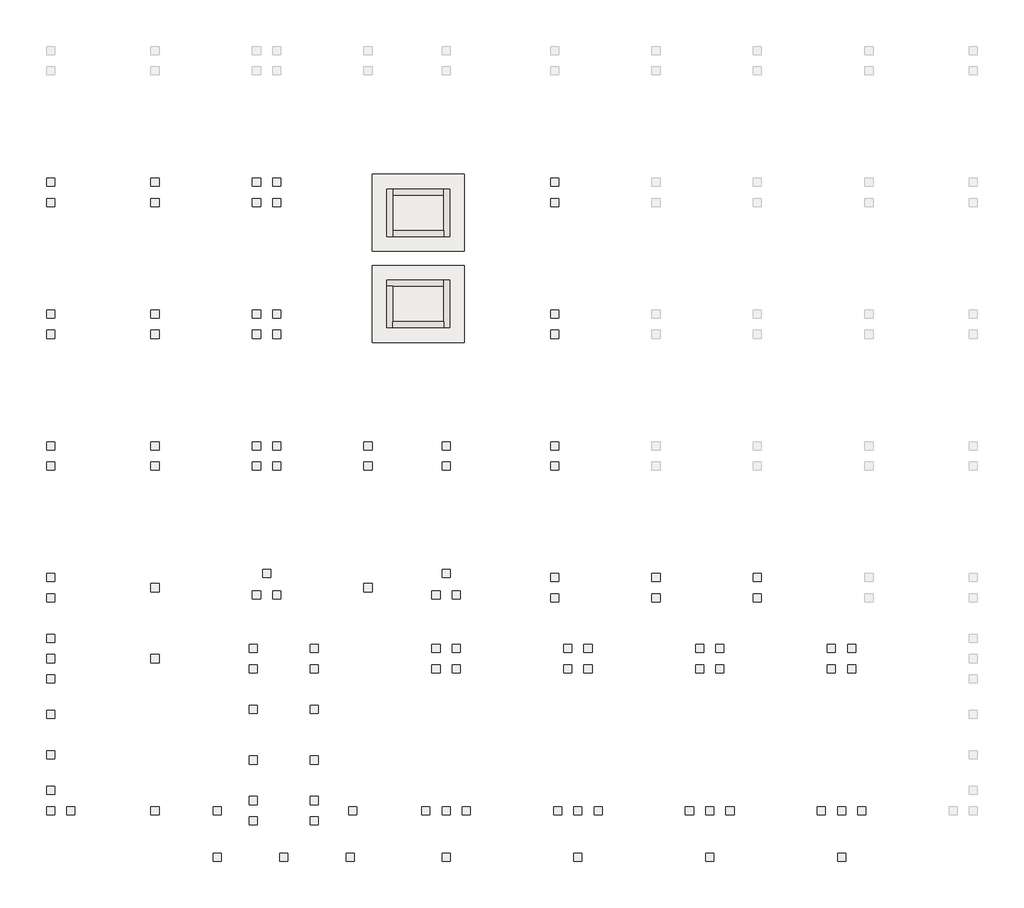
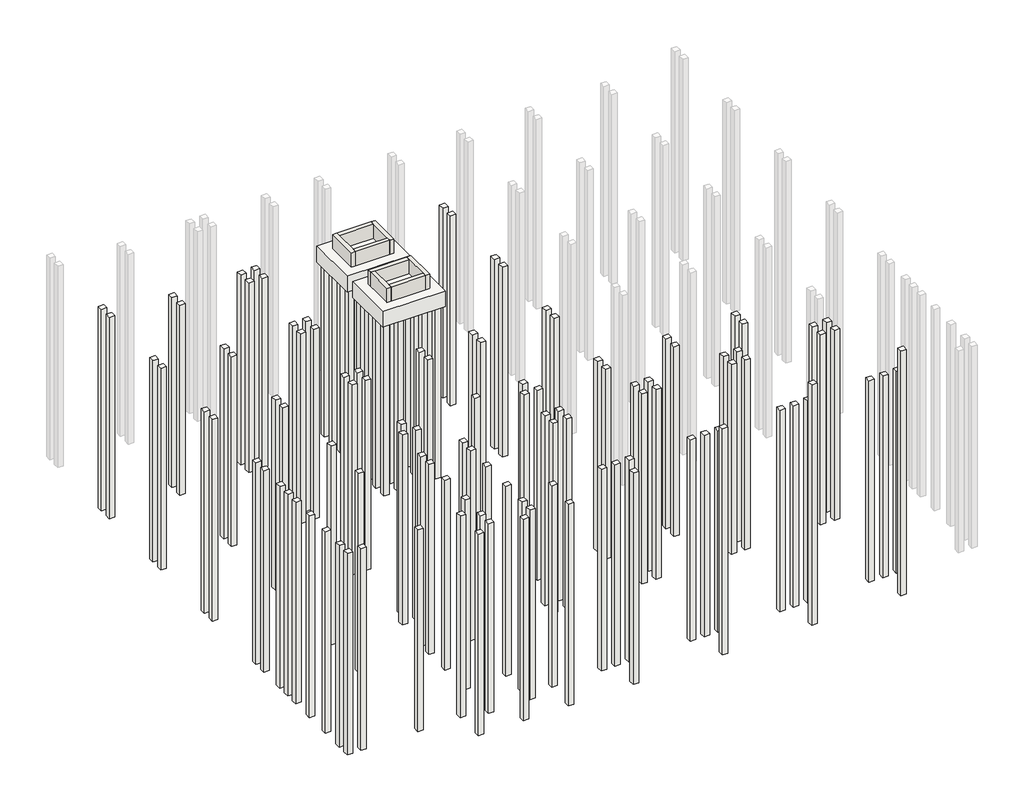
# Not in any storey, part 1 of 2: 143 slabs, 8 walls.
# Revit data of these elements (continued)
# Type "NLRS_16_SFO_LB_funderingspoer meerpaals beton ihwg-MMBC-SH_gen_rsf : funderingspoer beton ihwg_gen__lift bxlxh 3800x4550x1200" (continued)
#   Structural Material = NLRS_f2_beton ihwg_gen_rsf
#   Keynote = ""
# Type "NLRS_17_SFO_TLB_funderingspaal geheid beton prefab-AV-MMBPC_gen_rsf : heipaal beton prefab_gen__bxh 400x400"
#   Export Type to IFC As = "IfcPile"
#   Type IfcGUID = "10$Kfo5uPCAOPJEOo5LE_W"
#   Type Comments = "prefab heipaal 400x400"
#   Model = " "
#   Manufacturer = " "
#   Description = "prefab heipaal 400x400"
#   Assembly Code = "17.21"
#   Width = 400 mm
#   Slanted Angle [instance default] = 0.00°
#   NLRS_S_draagvermogen_trek [instance default] = 0.00 kN
#   NLRS_S_draagvermogen_druk [instance default] = 0.00 kN
#   NLRS_C_lengte [instance default] = 1660 mm
#   NLRS_C_hoogte = 400 mm
#   NLRS_C_breedte = 400 mm
#   Height [instance default] = 1660 mm
#   Length [instance default] = 1660 mm
#   Angle [instance default] = 0.00°
#   Slanted [instance default] = 0
#   Structural Material = NLRS_f2_beton prefab_gen_rsf
#   Keynote = ""
# Type "NLRS_16_WA_beton ihw 300_gen_rsf"
#   Keynote = ""
#   Export Type to IFC As = "IfcWall"
#   Type IfcGUID = "3S1HfGygHC08_ZXeiJ7DHR"
#   Description = "buitenwand beton ihw, generiek"
#   Assembly Code = "16.23"
#   Layers, outside or top first: 300 mm "NLRS_f2_beton ihwg_gen_rsf" (function 1)
# Element 1 (IfcSlab, "NLRS_16_SFO_LB_funderingspoer meerpaals beton ihwg-MMBC-SH_gen_rsf : funderingspoer beton ihwg_gen__lift bxlxh 3800x4550x1200")
#   IfcGUID = "22y6L5gAz9AR8RjJaZzOwK"
#   Height = 1200 mm
#   Depth = 0 mm
#   IsExternal = yes
#   LoadBearing = yes
#   Phase Created = NLRS_nieuw
#   Materials on its faces: "NLRS_f2_beton ihwg_gen_rsf"
# Element 2 (IfcSlab, "NLRS_16_SFO_LB_funderingspoer meerpaals beton ihwg-MMBC-SH_gen_rsf : funderingspoer beton ihwg_gen__lift bxlxh 3800x4550x1200")
#   IfcGUID = "22y6L5gAz9AR8RjJaZzOui"
#   Height = 1200 mm
#   Depth = 0 mm
#   IsExternal = yes
#   LoadBearing = yes
#   Phase Created = NLRS_nieuw
#   Materials on its faces: "NLRS_f2_beton ihwg_gen_rsf"
# Element 3 (IfcSlab, "NLRS_17_SFO_TLB_funderingspaal geheid beton prefab-AV-MMBPC_gen_rsf : heipaal beton prefab_gen__bxh 400x400")
#   IfcGUID = "10$Kfo5uPCAOPJEOo5LEvz"
#   Slanted Angle = 0.00°
#   NLRS_S_draagvermogen_trek = 0.00 kN
#   NLRS_S_draagvermogen_druk = 0.00 kN
#   Angle = 0.00°
#   IsExternal = yes
#   LoadBearing = yes
#   Slanted = 0
#   Phase Created = NLRS_nieuw
#   Materials on its faces: "NLRS_f2_beton prefab_gen_rsf"
# Element 4 (IfcSlab, "NLRS_17_SFO_TLB_funderingspaal geheid beton prefab-AV-MMBPC_gen_rsf : heipaal beton prefab_gen__bxh 400x400")
#   IfcGUID = "10$Kfo5uPCAOPJEOo5LEuK"
#   Slanted Angle = 0.00°
#   NLRS_S_draagvermogen_trek = 0.00 kN
#   NLRS_S_draagvermogen_druk = 0.00 kN
#   Angle = 0.00°
#   IsExternal = yes
#   LoadBearing = yes
#   Slanted = 0
#   Phase Created = NLRS_nieuw
#   Materials on its faces: "NLRS_f2_beton prefab_gen_rsf"
# Element 5 (IfcSlab, "NLRS_17_SFO_TLB_funderingspaal geheid beton prefab-AV-MMBPC_gen_rsf : heipaal beton prefab_gen__bxh 400x400")
#   IfcGUID = "10$Kfo5uPCAOPJEOo5LEuY"
#   Slanted Angle = 0.00°
#   NLRS_S_draagvermogen_trek = 0.00 kN
#   NLRS_S_draagvermogen_druk = 0.00 kN
#   Angle = 0.00°
#   IsExternal = yes
#   LoadBearing = yes
#   Slanted = 0
#   Phase Created = NLRS_nieuw
#   Materials on its faces: "NLRS_f2_beton prefab_gen_rsf"
# Element 6 (IfcSlab, "NLRS_17_SFO_TLB_funderingspaal geheid beton prefab-AV-MMBPC_gen_rsf : heipaal beton prefab_gen__bxh 400x400")
#   IfcGUID = "10$Kfo5uPCAOPJEOo5LEu$"
#   Slanted Angle = 0.00°
#   NLRS_S_draagvermogen_trek = 0.00 kN
#   NLRS_S_draagvermogen_druk = 0.00 kN
#   Angle = 0.00°
#   IsExternal = yes
#   LoadBearing = yes
#   Slanted = 0
#   Phase Created = NLRS_nieuw
#   Materials on its faces: "NLRS_f2_beton prefab_gen_rsf"
# Element 7 (IfcSlab, "NLRS_17_SFO_TLB_funderingspaal geheid beton prefab-AV-MMBPC_gen_rsf : heipaal beton prefab_gen__bxh 400x400")
#   IfcGUID = "10$Kfo5uPCAOPJEOo5LEun"
#   Slanted Angle = 0.00°
#   NLRS_S_draagvermogen_trek = 0.00 kN
#   NLRS_S_draagvermogen_druk = 0.00 kN
#   Angle = 0.00°
#   IsExternal = yes
#   LoadBearing = yes
#   Slanted = 0
#   Phase Created = NLRS_nieuw
#   Materials on its faces: "NLRS_f2_beton prefab_gen_rsf"
# Element 8 (IfcSlab, "NLRS_17_SFO_TLB_funderingspaal geheid beton prefab-AV-MMBPC_gen_rsf : heipaal beton prefab_gen__bxh 400x400")
#   IfcGUID = "10$Kfo5uPCAOPJEOo5LEtC"
#   Slanted Angle = 0.00°
#   NLRS_S_draagvermogen_trek = 0.00 kN
#   NLRS_S_draagvermogen_druk = 0.00 kN
#   Angle = 0.00°
#   IsExternal = yes
#   LoadBearing = yes
#   Slanted = 0
#   Phase Created = NLRS_nieuw
#   Materials on its faces: "NLRS_f2_beton prefab_gen_rsf"
# Element 9 (IfcSlab, "NLRS_17_SFO_TLB_funderingspaal geheid beton prefab-AV-MMBPC_gen_rsf : heipaal beton prefab_gen__bxh 400x400")
#   IfcGUID = "10$Kfo5uPCAOPJEOo5LEtE"
#   Slanted Angle = 0.00°
#   NLRS_S_draagvermogen_trek = 0.00 kN
#   NLRS_S_draagvermogen_druk = 0.00 kN
#   Angle = 0.00°
#   IsExternal = yes
#   LoadBearing = yes
#   Slanted = 0
#   Phase Created = NLRS_nieuw
#   Materials on its faces: "NLRS_f2_beton prefab_gen_rsf"
# Element 10 (IfcSlab, "NLRS_17_SFO_TLB_funderingspaal geheid beton prefab-AV-MMBPC_gen_rsf : heipaal beton prefab_gen__bxh 400x400")
#   IfcGUID = "10$Kfo5uPCAOPJEOo5LEtR"
#   Slanted Angle = 0.00°
#   NLRS_S_draagvermogen_trek = 0.00 kN
#   NLRS_S_draagvermogen_druk = 0.00 kN
#   Angle = 0.00°
#   IsExternal = yes
#   LoadBearing = yes
#   Slanted = 0
#   Phase Created = NLRS_nieuw
#   Materials on its faces: "NLRS_f2_beton prefab_gen_rsf"
# Element 11 (IfcSlab, "NLRS_17_SFO_TLB_funderingspaal geheid beton prefab-AV-MMBPC_gen_rsf : heipaal beton prefab_gen__bxh 400x400")
#   IfcGUID = "10$Kfo5uPCAOPJEOo5LEtT"
#   Slanted Angle = 0.00°
#   NLRS_S_draagvermogen_trek = 0.00 kN
#   NLRS_S_draagvermogen_druk = 0.00 kN
#   Angle = 0.00°
#   IsExternal = yes
#   LoadBearing = yes
#   Slanted = 0
#   Phase Created = NLRS_nieuw
#   Materials on its faces: "NLRS_f2_beton prefab_gen_rsf"
# Element 12 (IfcSlab, "NLRS_17_SFO_TLB_funderingspaal geheid beton prefab-AV-MMBPC_gen_rsf : heipaal beton prefab_gen__bxh 400x400")
#   IfcGUID = "10$Kfo5uPCAOPJEOo5LEte"
#   Slanted Angle = 0.00°
#   NLRS_S_draagvermogen_trek = 0.00 kN
#   NLRS_S_draagvermogen_druk = 0.00 kN
#   Angle = 0.00°
#   IsExternal = yes
#   LoadBearing = yes
#   Slanted = 0
#   Phase Created = NLRS_nieuw
#   Materials on its faces: "NLRS_f2_beton prefab_gen_rsf"
# Element 13 (IfcSlab, "NLRS_17_SFO_TLB_funderingspaal geheid beton prefab-AV-MMBPC_gen_rsf : heipaal beton prefab_gen__bxh 400x400")
#   IfcGUID = "10$Kfo5uPCAOPJEOo5LEtg"
#   Slanted Angle = 0.00°
#   NLRS_S_draagvermogen_trek = 0.00 kN
#   NLRS_S_draagvermogen_druk = 0.00 kN
#   Angle = 0.00°
#   IsExternal = yes
#   LoadBearing = yes
#   Slanted = 0
#   Phase Created = NLRS_nieuw
#   Materials on its faces: "NLRS_f2_beton prefab_gen_rsf"
# Element 14 (IfcSlab, "NLRS_17_SFO_TLB_funderingspaal geheid beton prefab-AV-MMBPC_gen_rsf : heipaal beton prefab_gen__bxh 400x400")
#   IfcGUID = "10$Kfo5uPCAOPJEOo5LEtb"
#   Slanted Angle = 0.00°
#   NLRS_S_draagvermogen_trek = 0.00 kN
#   NLRS_S_draagvermogen_druk = 0.00 kN
#   Angle = 0.00°
#   IsExternal = yes
#   LoadBearing = yes
#   Slanted = 0
#   Phase Created = NLRS_nieuw
#   Materials on its faces: "NLRS_f2_beton prefab_gen_rsf"
# Element 15 (IfcSlab, "NLRS_17_SFO_TLB_funderingspaal geheid beton prefab-AV-MMBPC_gen_rsf : heipaal beton prefab_gen__bxh 400x400")
#   IfcGUID = "10$Kfo5uPCAOPJEOo5LEtd"
#   Slanted Angle = 0.00°
#   NLRS_S_draagvermogen_trek = 0.00 kN
#   NLRS_S_draagvermogen_druk = 0.00 kN
#   Angle = 0.00°
#   IsExternal = yes
#   LoadBearing = yes
#   Slanted = 0
#   Phase Created = NLRS_nieuw
#   Materials on its faces: "NLRS_f2_beton prefab_gen_rsf"
# Element 16 (IfcSlab, "NLRS_17_SFO_TLB_funderingspaal geheid beton prefab-AV-MMBPC_gen_rsf : heipaal beton prefab_gen__bxh 400x400")
#   IfcGUID = "10$Kfo5uPCAOPJEOo5LEsp"
#   Slanted Angle = 0.00°
#   NLRS_S_draagvermogen_trek = 0.00 kN
#   NLRS_S_draagvermogen_druk = 0.00 kN
#   Angle = 0.00°
#   IsExternal = yes
#   LoadBearing = yes
#   Slanted = 0
#   Phase Created = NLRS_nieuw
#   Materials on its faces: "NLRS_f2_beton prefab_gen_rsf"
# Element 17 (IfcSlab, "NLRS_17_SFO_TLB_funderingspaal geheid beton prefab-AV-MMBPC_gen_rsf : heipaal beton prefab_gen__bxh 400x400")
#   IfcGUID = "10$Kfo5uPCAOPJEOo5LEsr"
#   Slanted Angle = 0.00°
#   NLRS_S_draagvermogen_trek = 0.00 kN
#   NLRS_S_draagvermogen_druk = 0.00 kN
#   Angle = 0.00°
#   IsExternal = yes
#   LoadBearing = yes
#   Slanted = 0
#   Phase Created = NLRS_nieuw
#   Materials on its faces: "NLRS_f2_beton prefab_gen_rsf"
# Element 18 (IfcSlab, "NLRS_17_SFO_TLB_funderingspaal geheid beton prefab-AV-MMBPC_gen_rsf : heipaal beton prefab_gen__bxh 400x400")
#   IfcGUID = "10$Kfo5uPCAOPJEOo5LEr0"
#   Slanted Angle = 0.00°
#   NLRS_S_draagvermogen_trek = 0.00 kN
#   NLRS_S_draagvermogen_druk = 0.00 kN
#   Angle = 0.00°
#   IsExternal = yes
#   LoadBearing = yes
#   Slanted = 0
#   Phase Created = NLRS_nieuw
#   Materials on its faces: "NLRS_f2_beton prefab_gen_rsf"
# Element 19 (IfcSlab, "NLRS_17_SFO_TLB_funderingspaal geheid beton prefab-AV-MMBPC_gen_rsf : heipaal beton prefab_gen__bxh 400x400")
#   IfcGUID = "10$Kfo5uPCAOPJEOo5LEr2"
#   Slanted Angle = 0.00°
#   NLRS_S_draagvermogen_trek = 0.00 kN
#   NLRS_S_draagvermogen_druk = 0.00 kN
#   Angle = 0.00°
#   IsExternal = yes
#   LoadBearing = yes
#   Slanted = 0
#   Phase Created = NLRS_nieuw
#   Materials on its faces: "NLRS_f2_beton prefab_gen_rsf"
# Element 20 (IfcSlab, "NLRS_17_SFO_TLB_funderingspaal geheid beton prefab-AV-MMBPC_gen_rsf : heipaal beton prefab_gen__bxh 400x400")
#   IfcGUID = "10$Kfo5uPCAOPJEOo5LErR"
#   Slanted Angle = 0.00°
#   NLRS_S_draagvermogen_trek = 0.00 kN
#   NLRS_S_draagvermogen_druk = 0.00 kN
#   Angle = 0.00°
#   IsExternal = yes
#   LoadBearing = yes
#   Slanted = 0
#   Phase Created = NLRS_nieuw
#   Materials on its faces: "NLRS_f2_beton prefab_gen_rsf"
# Element 21 (IfcSlab, "NLRS_17_SFO_TLB_funderingspaal geheid beton prefab-AV-MMBPC_gen_rsf : heipaal beton prefab_gen__bxh 400x400")
#   IfcGUID = "10$Kfo5uPCAOPJEOo5LErT"
#   Slanted Angle = 0.00°
#   NLRS_S_draagvermogen_trek = 0.00 kN
#   NLRS_S_draagvermogen_druk = 0.00 kN
#   Angle = 0.00°
#   IsExternal = yes
#   LoadBearing = yes
#   Slanted = 0
#   Phase Created = NLRS_nieuw
#   Materials on its faces: "NLRS_f2_beton prefab_gen_rsf"
# Element 22 (IfcSlab, "NLRS_17_SFO_TLB_funderingspaal geheid beton prefab-AV-MMBPC_gen_rsf : heipaal beton prefab_gen__bxh 400x400")
#   IfcGUID = "10$Kfo5uPCAOPJEOo5LErd"
#   Slanted Angle = 0.00°
#   NLRS_S_draagvermogen_trek = 0.00 kN
#   NLRS_S_draagvermogen_druk = 0.00 kN
#   Angle = 0.00°
#   IsExternal = yes
#   LoadBearing = yes
#   Slanted = 0
#   Phase Created = NLRS_nieuw
#   Materials on its faces: "NLRS_f2_beton prefab_gen_rsf"
# Element 23 (IfcSlab, "NLRS_17_SFO_TLB_funderingspaal geheid beton prefab-AV-MMBPC_gen_rsf : heipaal beton prefab_gen__bxh 400x400")
#   IfcGUID = "10$Kfo5uPCAOPJEOo5LErv"
#   Slanted Angle = 0.00°
#   NLRS_S_draagvermogen_trek = 0.00 kN
#   NLRS_S_draagvermogen_druk = 0.00 kN
#   Angle = 0.00°
#   IsExternal = yes
#   LoadBearing = yes
#   Slanted = 0
#   Phase Created = NLRS_nieuw
#   Materials on its faces: "NLRS_f2_beton prefab_gen_rsf"
# Element 24 (IfcSlab, "NLRS_17_SFO_TLB_funderingspaal geheid beton prefab-AV-MMBPC_gen_rsf : heipaal beton prefab_gen__bxh 400x400")
#   IfcGUID = "10$Kfo5uPCAOPJEOo5LEq5"
#   Slanted Angle = 0.00°
#   NLRS_S_draagvermogen_trek = 0.00 kN
#   NLRS_S_draagvermogen_druk = 0.00 kN
#   Angle = 0.00°
#   IsExternal = yes
#   LoadBearing = yes
#   Slanted = 0
#   Phase Created = NLRS_nieuw
#   Materials on its faces: "NLRS_f2_beton prefab_gen_rsf"
# Element 25 (IfcSlab, "NLRS_17_SFO_TLB_funderingspaal geheid beton prefab-AV-MMBPC_gen_rsf : heipaal beton prefab_gen__bxh 400x400")
#   IfcGUID = "10$Kfo5uPCAOPJEOo5LEq7"
#   Slanted Angle = 0.00°
#   NLRS_S_draagvermogen_trek = 0.00 kN
#   NLRS_S_draagvermogen_druk = 0.00 kN
#   Angle = 0.00°
#   IsExternal = yes
#   LoadBearing = yes
#   Slanted = 0
#   Phase Created = NLRS_nieuw
#   Materials on its faces: "NLRS_f2_beton prefab_gen_rsf"
# Element 26 (IfcSlab, "NLRS_17_SFO_TLB_funderingspaal geheid beton prefab-AV-MMBPC_gen_rsf : heipaal beton prefab_gen__bxh 400x400")
#   IfcGUID = "10$Kfo5uPCAOPJEOo5LEqa"
#   Slanted Angle = 0.00°
#   NLRS_S_draagvermogen_trek = 0.00 kN
#   NLRS_S_draagvermogen_druk = 0.00 kN
#   Angle = 0.00°
#   IsExternal = yes
#   LoadBearing = yes
#   Slanted = 0
#   Phase Created = NLRS_nieuw
#   Materials on its faces: "NLRS_f2_beton prefab_gen_rsf"
# Element 27 (IfcSlab, "NLRS_17_SFO_TLB_funderingspaal geheid beton prefab-AV-MMBPC_gen_rsf : heipaal beton prefab_gen__bxh 400x400")
#   IfcGUID = "10$Kfo5uPCAOPJEOo5LEqc"
#   Slanted Angle = 0.00°
#   NLRS_S_draagvermogen_trek = 0.00 kN
#   NLRS_S_draagvermogen_druk = 0.00 kN
#   Angle = 0.00°
#   IsExternal = yes
#   LoadBearing = yes
#   Slanted = 0
#   Phase Created = NLRS_nieuw
#   Materials on its faces: "NLRS_f2_beton prefab_gen_rsf"
# Element 28 (IfcSlab, "NLRS_17_SFO_TLB_funderingspaal geheid beton prefab-AV-MMBPC_gen_rsf : heipaal beton prefab_gen__bxh 400x400")
#   IfcGUID = "10$Kfo5uPCAOPJEOo5LEqy"
#   Slanted Angle = 0.00°
#   NLRS_S_draagvermogen_trek = 0.00 kN
#   NLRS_S_draagvermogen_druk = 0.00 kN
#   Angle = 0.00°
#   IsExternal = yes
#   LoadBearing = yes
#   Slanted = 0
#   Phase Created = NLRS_nieuw
#   Materials on its faces: "NLRS_f2_beton prefab_gen_rsf"
# Element 29 (IfcSlab, "NLRS_17_SFO_TLB_funderingspaal geheid beton prefab-AV-MMBPC_gen_rsf : heipaal beton prefab_gen__bxh 400x400")
#   IfcGUID = "10$Kfo5uPCAOPJEOo5LEq_"
#   Slanted Angle = 0.00°
#   NLRS_S_draagvermogen_trek = 0.00 kN
#   NLRS_S_draagvermogen_druk = 0.00 kN
#   Angle = 0.00°
#   IsExternal = yes
#   LoadBearing = yes
#   Slanted = 0
#   Phase Created = NLRS_nieuw
#   Materials on its faces: "NLRS_f2_beton prefab_gen_rsf"
# Element 30 (IfcSlab, "NLRS_17_SFO_TLB_funderingspaal geheid beton prefab-AV-MMBPC_gen_rsf : heipaal beton prefab_gen__bxh 400x400")
#   IfcGUID = "10$Kfo5uPCAOPJEOo5LEpB"
#   Slanted Angle = 0.00°
#   NLRS_S_draagvermogen_trek = 0.00 kN
#   NLRS_S_draagvermogen_druk = 0.00 kN
#   Angle = 0.00°
#   IsExternal = yes
#   LoadBearing = yes
#   Slanted = 0
#   Phase Created = NLRS_nieuw
#   Materials on its faces: "NLRS_f2_beton prefab_gen_rsf"
# Element 31 (IfcSlab, "NLRS_17_SFO_TLB_funderingspaal geheid beton prefab-AV-MMBPC_gen_rsf : heipaal beton prefab_gen__bxh 400x400")
#   IfcGUID = "10$Kfo5uPCAOPJEOo5LEpD"
#   Slanted Angle = 0.00°
#   NLRS_S_draagvermogen_trek = 0.00 kN
#   NLRS_S_draagvermogen_druk = 0.00 kN
#   Angle = 0.00°
#   IsExternal = yes
#   LoadBearing = yes
#   Slanted = 0
#   Phase Created = NLRS_nieuw
#   Materials on its faces: "NLRS_f2_beton prefab_gen_rsf"
# Element 32 (IfcSlab, "NLRS_17_SFO_TLB_funderingspaal geheid beton prefab-AV-MMBPC_gen_rsf : heipaal beton prefab_gen__bxh 400x400")
#   IfcGUID = "10$Kfo5uPCAOPJEOo5LEp3"
#   Slanted Angle = 0.00°
#   NLRS_S_draagvermogen_trek = 0.00 kN
#   NLRS_S_draagvermogen_druk = 0.00 kN
#   Angle = 0.00°
#   IsExternal = yes
#   LoadBearing = yes
#   Slanted = 0
#   Phase Created = NLRS_nieuw
#   Materials on its faces: "NLRS_f2_beton prefab_gen_rsf"
# Element 33 (IfcSlab, "NLRS_17_SFO_TLB_funderingspaal geheid beton prefab-AV-MMBPC_gen_rsf : heipaal beton prefab_gen__bxh 400x400")
#   IfcGUID = "10$Kfo5uPCAOPJEOo5LEp5"
#   Slanted Angle = 0.00°
#   NLRS_S_draagvermogen_trek = 0.00 kN
#   NLRS_S_draagvermogen_druk = 0.00 kN
#   Angle = 0.00°
#   IsExternal = yes
#   LoadBearing = yes
#   Slanted = 0
#   Phase Created = NLRS_nieuw
#   Materials on its faces: "NLRS_f2_beton prefab_gen_rsf"
# Element 34 (IfcSlab, "NLRS_17_SFO_TLB_funderingspaal geheid beton prefab-AV-MMBPC_gen_rsf : heipaal beton prefab_gen__bxh 400x400")
#   IfcGUID = "10$Kfo5uPCAOPJEOo5LEpG"
#   Slanted Angle = 0.00°
#   NLRS_S_draagvermogen_trek = 0.00 kN
#   NLRS_S_draagvermogen_druk = 0.00 kN
#   Angle = 0.00°
#   IsExternal = yes
#   LoadBearing = yes
#   Slanted = 0
#   Phase Created = NLRS_nieuw
#   Materials on its faces: "NLRS_f2_beton prefab_gen_rsf"
# Element 35 (IfcSlab, "NLRS_17_SFO_TLB_funderingspaal geheid beton prefab-AV-MMBPC_gen_rsf : heipaal beton prefab_gen__bxh 400x400")
#   IfcGUID = "10$Kfo5uPCAOPJEOo5LEpI"
#   Slanted Angle = 0.00°
#   NLRS_S_draagvermogen_trek = 0.00 kN
#   NLRS_S_draagvermogen_druk = 0.00 kN
#   Angle = 0.00°
#   IsExternal = yes
#   LoadBearing = yes
#   Slanted = 0
#   Phase Created = NLRS_nieuw
#   Materials on its faces: "NLRS_f2_beton prefab_gen_rsf"
# Element 36 (IfcSlab, "NLRS_17_SFO_TLB_funderingspaal geheid beton prefab-AV-MMBPC_gen_rsf : heipaal beton prefab_gen__bxh 400x400")
#   IfcGUID = "10$Kfo5uPCAOPJEOo5LEpe"
#   Slanted Angle = 0.00°
#   NLRS_S_draagvermogen_trek = 0.00 kN
#   NLRS_S_draagvermogen_druk = 0.00 kN
#   Angle = 0.00°
#   IsExternal = yes
#   LoadBearing = yes
#   Slanted = 0
#   Phase Created = NLRS_nieuw
#   Materials on its faces: "NLRS_f2_beton prefab_gen_rsf"
# Element 37 (IfcSlab, "NLRS_17_SFO_TLB_funderingspaal geheid beton prefab-AV-MMBPC_gen_rsf : heipaal beton prefab_gen__bxh 400x400")
#   IfcGUID = "10$Kfo5uPCAOPJEOo5LEpg"
#   Slanted Angle = 0.00°
#   NLRS_S_draagvermogen_trek = 0.00 kN
#   NLRS_S_draagvermogen_druk = 0.00 kN
#   Angle = 0.00°
#   IsExternal = yes
#   LoadBearing = yes
#   Slanted = 0
#   Phase Created = NLRS_nieuw
#   Materials on its faces: "NLRS_f2_beton prefab_gen_rsf"
# Element 38 (IfcSlab, "NLRS_17_SFO_TLB_funderingspaal geheid beton prefab-AV-MMBPC_gen_rsf : heipaal beton prefab_gen__bxh 400x400")
#   IfcGUID = "10$Kfo5uPCAOPJEOo5LEoA"
#   Slanted Angle = 0.00°
#   NLRS_S_draagvermogen_trek = 0.00 kN
#   NLRS_S_draagvermogen_druk = 0.00 kN
#   Angle = 0.00°
#   IsExternal = yes
#   LoadBearing = yes
#   Slanted = 0
#   Phase Created = NLRS_nieuw
#   Materials on its faces: "NLRS_f2_beton prefab_gen_rsf"
# Element 39 (IfcSlab, "NLRS_17_SFO_TLB_funderingspaal geheid beton prefab-AV-MMBPC_gen_rsf : heipaal beton prefab_gen__bxh 400x400")
#   IfcGUID = "10$Kfo5uPCAOPJEOo5LEoC"
#   Slanted Angle = 0.00°
#   NLRS_S_draagvermogen_trek = 0.00 kN
#   NLRS_S_draagvermogen_druk = 0.00 kN
#   Angle = 0.00°
#   IsExternal = yes
#   LoadBearing = yes
#   Slanted = 0
#   Phase Created = NLRS_nieuw
#   Materials on its faces: "NLRS_f2_beton prefab_gen_rsf"
# Element 40 (IfcSlab, "NLRS_17_SFO_TLB_funderingspaal geheid beton prefab-AV-MMBPC_gen_rsf : heipaal beton prefab_gen__bxh 400x400")
#   IfcGUID = "10$Kfo5uPCAOPJEOo5LEo2"
#   Slanted Angle = 0.00°
#   NLRS_S_draagvermogen_trek = 0.00 kN
#   NLRS_S_draagvermogen_druk = 0.00 kN
#   Angle = 0.00°
#   IsExternal = yes
#   LoadBearing = yes
#   Slanted = 0
#   Phase Created = NLRS_nieuw
#   Materials on its faces: "NLRS_f2_beton prefab_gen_rsf"
# Element 41 (IfcSlab, "NLRS_17_SFO_TLB_funderingspaal geheid beton prefab-AV-MMBPC_gen_rsf : heipaal beton prefab_gen__bxh 400x400")
#   IfcGUID = "10$Kfo5uPCAOPJEOo5LEo4"
#   Slanted Angle = 0.00°
#   NLRS_S_draagvermogen_trek = 0.00 kN
#   NLRS_S_draagvermogen_druk = 0.00 kN
#   Angle = 0.00°
#   IsExternal = yes
#   LoadBearing = yes
#   Slanted = 0
#   Phase Created = NLRS_nieuw
#   Materials on its faces: "NLRS_f2_beton prefab_gen_rsf"
# Element 42 (IfcSlab, "NLRS_17_SFO_TLB_funderingspaal geheid beton prefab-AV-MMBPC_gen_rsf : heipaal beton prefab_gen__bxh 400x400")
#   IfcGUID = "10$Kfo5uPCAOPJEOo5LEoV"
#   Slanted Angle = 0.00°
#   NLRS_S_draagvermogen_trek = 0.00 kN
#   NLRS_S_draagvermogen_druk = 0.00 kN
#   Angle = 0.00°
#   IsExternal = yes
#   LoadBearing = yes
#   Slanted = 0
#   Phase Created = NLRS_nieuw
#   Materials on its faces: "NLRS_f2_beton prefab_gen_rsf"
# Element 43 (IfcSlab, "NLRS_17_SFO_TLB_funderingspaal geheid beton prefab-AV-MMBPC_gen_rsf : heipaal beton prefab_gen__bxh 400x400")
#   IfcGUID = "10$Kfo5uPCAOPJEOo5LEoH"
#   Slanted Angle = 0.00°
#   NLRS_S_draagvermogen_trek = 0.00 kN
#   NLRS_S_draagvermogen_druk = 0.00 kN
#   Angle = 0.00°
#   IsExternal = yes
#   LoadBearing = yes
#   Slanted = 0
#   Phase Created = NLRS_nieuw
#   Materials on its faces: "NLRS_f2_beton prefab_gen_rsf"
# Element 44 (IfcSlab, "NLRS_17_SFO_TLB_funderingspaal geheid beton prefab-AV-MMBPC_gen_rsf : heipaal beton prefab_gen__bxh 400x400")
#   IfcGUID = "10$Kfo5uPCAOPJEOo5LEoN"
#   Slanted Angle = 0.00°
#   NLRS_S_draagvermogen_trek = 0.00 kN
#   NLRS_S_draagvermogen_druk = 0.00 kN
#   Angle = 0.00°
#   IsExternal = yes
#   LoadBearing = yes
#   Slanted = 0
#   Phase Created = NLRS_nieuw
#   Materials on its faces: "NLRS_f2_beton prefab_gen_rsf"
# Element 45 (IfcSlab, "NLRS_17_SFO_TLB_funderingspaal geheid beton prefab-AV-MMBPC_gen_rsf : heipaal beton prefab_gen__bxh 400x400")
#   IfcGUID = "10$Kfo5uPCAOPJEOo5LEof"
#   Slanted Angle = 0.00°
#   NLRS_S_draagvermogen_trek = 0.00 kN
#   NLRS_S_draagvermogen_druk = 0.00 kN
#   Angle = 0.00°
#   IsExternal = yes
#   LoadBearing = yes
#   Slanted = 0
#   Phase Created = NLRS_nieuw
#   Materials on its faces: "NLRS_f2_beton prefab_gen_rsf"
# Element 46 (IfcSlab, "NLRS_17_SFO_TLB_funderingspaal geheid beton prefab-AV-MMBPC_gen_rsf : heipaal beton prefab_gen__bxh 400x400")
#   IfcGUID = "10$Kfo5uPCAOPJEOo5LEoc"
#   Slanted Angle = 0.00°
#   NLRS_S_draagvermogen_trek = 0.00 kN
#   NLRS_S_draagvermogen_druk = 0.00 kN
#   Angle = 0.00°
#   IsExternal = yes
#   LoadBearing = yes
#   Slanted = 0
#   Phase Created = NLRS_nieuw
#   Materials on its faces: "NLRS_f2_beton prefab_gen_rsf"
# Element 47 (IfcSlab, "NLRS_17_SFO_TLB_funderingspaal geheid beton prefab-AV-MMBPC_gen_rsf : heipaal beton prefab_gen__bxh 400x400")
#   IfcGUID = "10$Kfo5uPCAOPJEOo5LEou"
#   Slanted Angle = 0.00°
#   NLRS_S_draagvermogen_trek = 0.00 kN
#   NLRS_S_draagvermogen_druk = 0.00 kN
#   Angle = 0.00°
#   IsExternal = yes
#   LoadBearing = yes
#   Slanted = 0
#   Phase Created = NLRS_nieuw
#   Materials on its faces: "NLRS_f2_beton prefab_gen_rsf"
# Element 48 (IfcSlab, "NLRS_17_SFO_TLB_funderingspaal geheid beton prefab-AV-MMBPC_gen_rsf : heipaal beton prefab_gen__bxh 400x400")
#   IfcGUID = "10$Kfo5uPCAOPJEOo5LEo_"
#   Slanted Angle = 0.00°
#   NLRS_S_draagvermogen_trek = 0.00 kN
#   NLRS_S_draagvermogen_druk = 0.00 kN
#   Angle = 0.00°
#   IsExternal = yes
#   LoadBearing = yes
#   Slanted = 0
#   Phase Created = NLRS_nieuw
#   Materials on its faces: "NLRS_f2_beton prefab_gen_rsf"
# Element 49 (IfcSlab, "NLRS_17_SFO_TLB_funderingspaal geheid beton prefab-AV-MMBPC_gen_rsf : heipaal beton prefab_gen__bxh 400x400")
#   IfcGUID = "10$Kfo5uPCAOPJEOo5LEom"
#   Slanted Angle = 0.00°
#   NLRS_S_draagvermogen_trek = 0.00 kN
#   NLRS_S_draagvermogen_druk = 0.00 kN
#   Angle = 0.00°
#   IsExternal = yes
#   LoadBearing = yes
#   Slanted = 0
#   Phase Created = NLRS_nieuw
#   Materials on its faces: "NLRS_f2_beton prefab_gen_rsf"
# Element 50 (IfcSlab, "NLRS_17_SFO_TLB_funderingspaal geheid beton prefab-AV-MMBPC_gen_rsf : heipaal beton prefab_gen__bxh 400x400")
#   IfcGUID = "10$Kfo5uPCAOPJEOo5LEnB"
#   Slanted Angle = 0.00°
#   NLRS_S_draagvermogen_trek = 0.00 kN
#   NLRS_S_draagvermogen_druk = 0.00 kN
#   Angle = 0.00°
#   IsExternal = yes
#   LoadBearing = yes
#   Slanted = 0
#   Phase Created = NLRS_nieuw
#   Materials on its faces: "NLRS_f2_beton prefab_gen_rsf"
# Element 51 (IfcSlab, "NLRS_17_SFO_TLB_funderingspaal geheid beton prefab-AV-MMBPC_gen_rsf : heipaal beton prefab_gen__bxh 400x400")
#   IfcGUID = "10$Kfo5uPCAOPJEOo5LEnF"
#   Slanted Angle = 0.00°
#   NLRS_S_draagvermogen_trek = 0.00 kN
#   NLRS_S_draagvermogen_druk = 0.00 kN
#   Angle = 0.00°
#   IsExternal = yes
#   LoadBearing = yes
#   Slanted = 0
#   Phase Created = NLRS_nieuw
#   Materials on its faces: "NLRS_f2_beton prefab_gen_rsf"
# Element 52 (IfcSlab, "NLRS_17_SFO_TLB_funderingspaal geheid beton prefab-AV-MMBPC_gen_rsf : heipaal beton prefab_gen__bxh 400x400")
#   IfcGUID = "10$Kfo5uPCAOPJEOo5LEn1"
#   Slanted Angle = 0.00°
#   NLRS_S_draagvermogen_trek = 0.00 kN
#   NLRS_S_draagvermogen_druk = 0.00 kN
#   Angle = 0.00°
#   IsExternal = yes
#   LoadBearing = yes
#   Slanted = 0
#   Phase Created = NLRS_nieuw
#   Materials on its faces: "NLRS_f2_beton prefab_gen_rsf"
# Element 53 (IfcSlab, "NLRS_17_SFO_TLB_funderingspaal geheid beton prefab-AV-MMBPC_gen_rsf : heipaal beton prefab_gen__bxh 400x400")
#   IfcGUID = "10$Kfo5uPCAOPJEOo5LEWk"
#   Slanted Angle = 0.00°
#   NLRS_S_draagvermogen_trek = 0.00 kN
#   NLRS_S_draagvermogen_druk = 0.00 kN
#   Angle = 0.00°
#   IsExternal = yes
#   LoadBearing = yes
#   Slanted = 0
#   Phase Created = NLRS_nieuw
#   Materials on its faces: "NLRS_f2_beton prefab_gen_rsf"
# Element 54 (IfcSlab, "NLRS_17_SFO_TLB_funderingspaal geheid beton prefab-AV-MMBPC_gen_rsf : heipaal beton prefab_gen__bxh 400x400")
#   IfcGUID = "10$Kfo5uPCAOPJEOo5LEWW"
#   Slanted Angle = 0.00°
#   NLRS_S_draagvermogen_trek = 0.00 kN
#   NLRS_S_draagvermogen_druk = 0.00 kN
#   Angle = 0.00°
#   IsExternal = yes
#   LoadBearing = yes
#   Slanted = 0
#   Phase Created = NLRS_nieuw
#   Materials on its faces: "NLRS_f2_beton prefab_gen_rsf"
# Element 55 (IfcSlab, "NLRS_17_SFO_TLB_funderingspaal geheid beton prefab-AV-MMBPC_gen_rsf : heipaal beton prefab_gen__bxh 400x400")
#   IfcGUID = "10$Kfo5uPCAOPJEOo5LEWY"
#   Slanted Angle = 0.00°
#   NLRS_S_draagvermogen_trek = 0.00 kN
#   NLRS_S_draagvermogen_druk = 0.00 kN
#   Angle = 0.00°
#   IsExternal = yes
#   LoadBearing = yes
#   Slanted = 0
#   Phase Created = NLRS_nieuw
#   Materials on its faces: "NLRS_f2_beton prefab_gen_rsf"
# Element 56 (IfcSlab, "NLRS_17_SFO_TLB_funderingspaal geheid beton prefab-AV-MMBPC_gen_rsf : heipaal beton prefab_gen__bxh 400x400")
#   IfcGUID = "10$Kfo5uPCAOPJEOo5LEWa"
#   Slanted Angle = 0.00°
#   NLRS_S_draagvermogen_trek = 0.00 kN
#   NLRS_S_draagvermogen_druk = 0.00 kN
#   Angle = 0.00°
#   IsExternal = yes
#   LoadBearing = yes
#   Slanted = 0
#   Phase Created = NLRS_nieuw
#   Materials on its faces: "NLRS_f2_beton prefab_gen_rsf"
# Element 57 (IfcSlab, "NLRS_17_SFO_TLB_funderingspaal geheid beton prefab-AV-MMBPC_gen_rsf : heipaal beton prefab_gen__bxh 400x400")
#   IfcGUID = "10$Kfo5uPCAOPJEOo5LEWp"
#   Slanted Angle = 0.00°
#   NLRS_S_draagvermogen_trek = 0.00 kN
#   NLRS_S_draagvermogen_druk = 0.00 kN
#   Angle = 0.00°
#   IsExternal = yes
#   LoadBearing = yes
#   Slanted = 0
#   Phase Created = NLRS_nieuw
#   Materials on its faces: "NLRS_f2_beton prefab_gen_rsf"
# Element 58 (IfcSlab, "NLRS_17_SFO_TLB_funderingspaal geheid beton prefab-AV-MMBPC_gen_rsf : heipaal beton prefab_gen__bxh 400x400")
#   IfcGUID = "10$Kfo5uPCAOPJEOo5LEWr"
#   Slanted Angle = 0.00°
#   NLRS_S_draagvermogen_trek = 0.00 kN
#   NLRS_S_draagvermogen_druk = 0.00 kN
#   Angle = 0.00°
#   IsExternal = yes
#   LoadBearing = yes
#   Slanted = 0
#   Phase Created = NLRS_nieuw
#   Materials on its faces: "NLRS_f2_beton prefab_gen_rsf"
# Element 59 (IfcSlab, "NLRS_17_SFO_TLB_funderingspaal geheid beton prefab-AV-MMBPC_gen_rsf : heipaal beton prefab_gen__bxh 400x400")
#   IfcGUID = "10$Kfo5uPCAOPJEOo5LEWt"
#   Slanted Angle = 0.00°
#   NLRS_S_draagvermogen_trek = 0.00 kN
#   NLRS_S_draagvermogen_druk = 0.00 kN
#   Angle = 0.00°
#   IsExternal = yes
#   LoadBearing = yes
#   Slanted = 0
#   Phase Created = NLRS_nieuw
#   Materials on its faces: "NLRS_f2_beton prefab_gen_rsf"
# Element 60 (IfcSlab, "NLRS_17_SFO_TLB_funderingspaal geheid beton prefab-AV-MMBPC_gen_rsf : heipaal beton prefab_gen__bxh 400x400")
#   IfcGUID = "10$Kfo5uPCAOPJEOo5LFV9"
#   Slanted Angle = 0.00°
#   NLRS_S_draagvermogen_trek = 0.00 kN
#   NLRS_S_draagvermogen_druk = 0.00 kN
#   Angle = 0.00°
#   IsExternal = yes
#   LoadBearing = yes
#   Slanted = 0
#   Phase Created = NLRS_nieuw
#   Materials on its faces: "NLRS_f2_beton prefab_gen_rsf"
# Element 61 (IfcSlab, "NLRS_17_SFO_TLB_funderingspaal geheid beton prefab-AV-MMBPC_gen_rsf : heipaal beton prefab_gen__bxh 400x400")
#   IfcGUID = "10$Kfo5uPCAOPJEOo5LFVh"
#   Slanted Angle = 0.00°
#   NLRS_S_draagvermogen_trek = 0.00 kN
#   NLRS_S_draagvermogen_druk = 0.00 kN
#   Angle = 0.00°
#   IsExternal = yes
#   LoadBearing = yes
#   Slanted = 0
#   Phase Created = NLRS_nieuw
#   Materials on its faces: "NLRS_f2_beton prefab_gen_rsf"
# Element 62 (IfcSlab, "NLRS_17_SFO_TLB_funderingspaal geheid beton prefab-AV-MMBPC_gen_rsf : heipaal beton prefab_gen__bxh 400x400")
#   IfcGUID = "10$Kfo5uPCAOPJEOo5LFNw"
#   Slanted Angle = 0.00°
#   NLRS_S_draagvermogen_trek = 0.00 kN
#   NLRS_S_draagvermogen_druk = 0.00 kN
#   Angle = 0.00°
#   IsExternal = yes
#   LoadBearing = yes
#   Slanted = 0
#   Phase Created = NLRS_nieuw
#   Materials on its faces: "NLRS_f2_beton prefab_gen_rsf"
# Element 63 (IfcSlab, "NLRS_17_SFO_TLB_funderingspaal geheid beton prefab-AV-MMBPC_gen_rsf : heipaal beton prefab_gen__bxh 400x400")
#   IfcGUID = "0NibaB7BP2RgdAc9dAk1VF"
#   Slanted Angle = 0.00°
#   NLRS_S_draagvermogen_trek = 0.00 kN
#   NLRS_S_draagvermogen_druk = 0.00 kN
#   Angle = 0.00°
#   IsExternal = yes
#   LoadBearing = yes
#   Slanted = 0
#   Phase Created = NLRS_nieuw
#   Materials on its faces: "NLRS_f2_beton prefab_gen_rsf"
# Element 64 (IfcSlab, "NLRS_17_SFO_TLB_funderingspaal geheid beton prefab-AV-MMBPC_gen_rsf : heipaal beton prefab_gen__bxh 400x400")
#   IfcGUID = "0NibaB7BP2RgdAc9dAk1UY"
#   Slanted Angle = 0.00°
#   NLRS_S_draagvermogen_trek = 0.00 kN
#   NLRS_S_draagvermogen_druk = 0.00 kN
#   Angle = 0.00°
#   IsExternal = yes
#   LoadBearing = yes
#   Slanted = 0
#   Phase Created = NLRS_nieuw
#   Materials on its faces: "NLRS_f2_beton prefab_gen_rsf"
# Element 65 (IfcSlab, "NLRS_17_SFO_TLB_funderingspaal geheid beton prefab-AV-MMBPC_gen_rsf : heipaal beton prefab_gen__bxh 400x400")
#   IfcGUID = "3loy75XKz2Rw4dS8JWiauf"
#   Slanted Angle = 0.00°
#   NLRS_S_draagvermogen_trek = 0.00 kN
#   NLRS_S_draagvermogen_druk = 0.00 kN
#   Angle = 0.00°
#   IsExternal = yes
#   LoadBearing = yes
#   Slanted = 0
#   Phase Created = NLRS_nieuw
#   Materials on its faces: "NLRS_f2_beton prefab_gen_rsf"
# Element 66 (IfcSlab, "NLRS_17_SFO_TLB_funderingspaal geheid beton prefab-AV-MMBPC_gen_rsf : heipaal beton prefab_gen__bxh 400x400")
#   IfcGUID = "3loy75XKz2Rw4dS8JWiaul"
#   Slanted Angle = 0.00°
#   NLRS_S_draagvermogen_trek = 0.00 kN
#   NLRS_S_draagvermogen_druk = 0.00 kN
#   Angle = 0.00°
#   IsExternal = yes
#   LoadBearing = yes
#   Slanted = 0
#   Phase Created = NLRS_nieuw
#   Materials on its faces: "NLRS_f2_beton prefab_gen_rsf"
# Element 67 (IfcSlab, "NLRS_17_SFO_TLB_funderingspaal geheid beton prefab-AV-MMBPC_gen_rsf : heipaal beton prefab_gen__bxh 400x400")
#   IfcGUID = "3loy75XKz2Rw4dS8JWiauj"
#   Slanted Angle = 0.00°
#   NLRS_S_draagvermogen_trek = 0.00 kN
#   NLRS_S_draagvermogen_druk = 0.00 kN
#   Angle = 0.00°
#   IsExternal = yes
#   LoadBearing = yes
#   Slanted = 0
#   Phase Created = NLRS_nieuw
#   Materials on its faces: "NLRS_f2_beton prefab_gen_rsf"
# Element 68 (IfcSlab, "NLRS_17_SFO_TLB_funderingspaal geheid beton prefab-AV-MMBPC_gen_rsf : heipaal beton prefab_gen__bxh 400x400")
#   IfcGUID = "3loy75XKz2Rw4dS8JWiam3"
#   Slanted Angle = 0.00°
#   NLRS_S_draagvermogen_trek = 0.00 kN
#   NLRS_S_draagvermogen_druk = 0.00 kN
#   Angle = 0.00°
#   IsExternal = yes
#   LoadBearing = yes
#   Slanted = 0
#   Phase Created = NLRS_nieuw
#   Materials on its faces: "NLRS_f2_beton prefab_gen_rsf"
# Element 69 (IfcSlab, "NLRS_17_SFO_TLB_funderingspaal geheid beton prefab-AV-MMBPC_gen_rsf : heipaal beton prefab_gen__bxh 400x400")
#   IfcGUID = "3loy75XKz2Rw4dS8JWiam1"
#   Slanted Angle = 0.00°
#   NLRS_S_draagvermogen_trek = 0.00 kN
#   NLRS_S_draagvermogen_druk = 0.00 kN
#   Angle = 0.00°
#   IsExternal = yes
#   LoadBearing = yes
#   Slanted = 0
#   Phase Created = NLRS_nieuw
#   Materials on its faces: "NLRS_f2_beton prefab_gen_rsf"
# Element 70 (IfcSlab, "NLRS_17_SFO_TLB_funderingspaal geheid beton prefab-AV-MMBPC_gen_rsf : heipaal beton prefab_gen__bxh 400x400")
#   IfcGUID = "3loy75XKz2Rw4dS8JWiapu"
#   Slanted Angle = 0.00°
#   NLRS_S_draagvermogen_trek = 0.00 kN
#   NLRS_S_draagvermogen_druk = 0.00 kN
#   Angle = 0.00°
#   IsExternal = yes
#   LoadBearing = yes
#   Slanted = 0
#   Phase Created = NLRS_nieuw
#   Materials on its faces: "NLRS_f2_beton prefab_gen_rsf"
# Element 71 (IfcSlab, "NLRS_17_SFO_TLB_funderingspaal geheid beton prefab-AV-MMBPC_gen_rsf : heipaal beton prefab_gen__bxh 400x400")
#   IfcGUID = "3loy75XKz2Rw4dS8JWiap_"
#   Slanted Angle = 0.00°
#   NLRS_S_draagvermogen_trek = 0.00 kN
#   NLRS_S_draagvermogen_druk = 0.00 kN
#   Angle = 0.00°
#   IsExternal = yes
#   LoadBearing = yes
#   Slanted = 0
#   Phase Created = NLRS_nieuw
#   Materials on its faces: "NLRS_f2_beton prefab_gen_rsf"
# Element 72 (IfcSlab, "NLRS_17_SFO_TLB_funderingspaal geheid beton prefab-AV-MMBPC_gen_rsf : heipaal beton prefab_gen__bxh 400x400")
#   IfcGUID = "3loy75XKz2Rw4dS8JWiaoR"
#   Slanted Angle = 0.00°
#   NLRS_S_draagvermogen_trek = 0.00 kN
#   NLRS_S_draagvermogen_druk = 0.00 kN
#   Angle = 0.00°
#   IsExternal = yes
#   LoadBearing = yes
#   Slanted = 0
#   Phase Created = NLRS_nieuw
#   Materials on its faces: "NLRS_f2_beton prefab_gen_rsf"
# Element 73 (IfcSlab, "NLRS_17_SFO_TLB_funderingspaal geheid beton prefab-AV-MMBPC_gen_rsf : heipaal beton prefab_gen__bxh 400x400")
#   IfcGUID = "3loy75XKz2Rw4dS8JWiaoP"
#   Slanted Angle = 0.00°
#   NLRS_S_draagvermogen_trek = 0.00 kN
#   NLRS_S_draagvermogen_druk = 0.00 kN
#   Angle = 0.00°
#   IsExternal = yes
#   LoadBearing = yes
#   Slanted = 0
#   Phase Created = NLRS_nieuw
#   Materials on its faces: "NLRS_f2_beton prefab_gen_rsf"
# Element 74 (IfcSlab, "NLRS_17_SFO_TLB_funderingspaal geheid beton prefab-AV-MMBPC_gen_rsf : heipaal beton prefab_gen__bxh 400x400")
#   IfcGUID = "0NibaB7BP2RgdAc9dAk1EY"
#   Slanted Angle = 0.00°
#   NLRS_S_draagvermogen_trek = 0.00 kN
#   NLRS_S_draagvermogen_druk = 0.00 kN
#   Angle = 0.00°
#   IsExternal = yes
#   LoadBearing = yes
#   Slanted = 0
#   Phase Created = NLRS_nieuw
#   Materials on its faces: "NLRS_f2_beton prefab_gen_rsf"
# Element 75 (IfcSlab, "NLRS_17_SFO_TLB_funderingspaal geheid beton prefab-AV-MMBPC_gen_rsf : heipaal beton prefab_gen__bxh 400x400")
#   IfcGUID = "0NibaB7BP2RgdAc9dAk1EP"
#   Slanted Angle = 0.00°
#   NLRS_S_draagvermogen_trek = 0.00 kN
#   NLRS_S_draagvermogen_druk = 0.00 kN
#   Angle = 0.00°
#   IsExternal = yes
#   LoadBearing = yes
#   Slanted = 0
#   Phase Created = NLRS_nieuw
#   Materials on its faces: "NLRS_f2_beton prefab_gen_rsf"
# Element 76 (IfcSlab, "NLRS_17_SFO_TLB_funderingspaal geheid beton prefab-AV-MMBPC_gen_rsf : heipaal beton prefab_gen__bxh 400x400")
#   IfcGUID = "0NibaB7BP2RgdAc9dAk1Di"
#   Slanted Angle = 0.00°
#   NLRS_S_draagvermogen_trek = 0.00 kN
#   NLRS_S_draagvermogen_druk = 0.00 kN
#   Angle = 0.00°
#   IsExternal = yes
#   LoadBearing = yes
#   Slanted = 0
#   Phase Created = NLRS_nieuw
#   Materials on its faces: "NLRS_f2_beton prefab_gen_rsf"
# Element 77 (IfcSlab, "NLRS_17_SFO_TLB_funderingspaal geheid beton prefab-AV-MMBPC_gen_rsf : heipaal beton prefab_gen__bxh 400x400")
#   IfcGUID = "0NibaB7BP2RgdAc9dAk1SD"
#   Slanted Angle = 0.00°
#   NLRS_S_draagvermogen_trek = 0.00 kN
#   NLRS_S_draagvermogen_druk = 0.00 kN
#   Angle = 0.00°
#   IsExternal = yes
#   LoadBearing = yes
#   Slanted = 0
#   Phase Created = NLRS_nieuw
#   Materials on its faces: "NLRS_f2_beton prefab_gen_rsf"
# Element 78 (IfcSlab, "NLRS_17_SFO_TLB_funderingspaal geheid beton prefab-AV-MMBPC_gen_rsf : heipaal beton prefab_gen__bxh 400x400")
#   IfcGUID = "0NibaB7BP2RgdAc9dAk6Zm"
#   Slanted Angle = 0.00°
#   NLRS_S_draagvermogen_trek = 0.00 kN
#   NLRS_S_draagvermogen_druk = 0.00 kN
#   Angle = 0.00°
#   IsExternal = yes
#   LoadBearing = yes
#   Slanted = 0
#   Phase Created = NLRS_nieuw
#   Materials on its faces: "NLRS_f2_beton prefab_gen_rsf"
# Element 79 (IfcSlab, "NLRS_17_SFO_TLB_funderingspaal geheid beton prefab-AV-MMBPC_gen_rsf : heipaal beton prefab_gen__bxh 400x400")
#   IfcGUID = "0NibaB7BP2RgdAc9dAk6ZH"
#   Slanted Angle = 0.00°
#   NLRS_S_draagvermogen_trek = 0.00 kN
#   NLRS_S_draagvermogen_druk = 0.00 kN
#   Angle = 0.00°
#   IsExternal = yes
#   LoadBearing = yes
#   Slanted = 0
#   Phase Created = NLRS_nieuw
#   Materials on its faces: "NLRS_f2_beton prefab_gen_rsf"
# Element 80 (IfcSlab, "NLRS_17_SFO_TLB_funderingspaal geheid beton prefab-AV-MMBPC_gen_rsf : heipaal beton prefab_gen__bxh 400x400")
#   IfcGUID = "0NibaB7BP2RgdAc9dAk6Y9"
#   Slanted Angle = 0.00°
#   NLRS_S_draagvermogen_trek = 0.00 kN
#   NLRS_S_draagvermogen_druk = 0.00 kN
#   Angle = 0.00°
#   IsExternal = yes
#   LoadBearing = yes
#   Slanted = 0
#   Phase Created = NLRS_nieuw
#   Materials on its faces: "NLRS_f2_beton prefab_gen_rsf"
# Element 81 (IfcSlab, "NLRS_17_SFO_TLB_funderingspaal geheid beton prefab-AV-MMBPC_gen_rsf : heipaal beton prefab_gen__bxh 400x400")
#   IfcGUID = "0NibaB7BP2RgdAc9dAk6Y7"
#   Slanted Angle = 0.00°
#   NLRS_S_draagvermogen_trek = 0.00 kN
#   NLRS_S_draagvermogen_druk = 0.00 kN
#   Angle = 0.00°
#   IsExternal = yes
#   LoadBearing = yes
#   Slanted = 0
#   Phase Created = NLRS_nieuw
#   Materials on its faces: "NLRS_f2_beton prefab_gen_rsf"
# Element 82 (IfcSlab, "NLRS_17_SFO_TLB_funderingspaal geheid beton prefab-AV-MMBPC_gen_rsf : heipaal beton prefab_gen__bxh 400x400")
#   IfcGUID = "0NibaB7BP2RgdAc9dAk6XN"
#   Slanted Angle = 0.00°
#   NLRS_S_draagvermogen_trek = 0.00 kN
#   NLRS_S_draagvermogen_druk = 0.00 kN
#   Angle = 0.00°
#   IsExternal = yes
#   LoadBearing = yes
#   Slanted = 0
#   Phase Created = NLRS_nieuw
#   Materials on its faces: "NLRS_f2_beton prefab_gen_rsf"
# Element 83 (IfcSlab, "NLRS_17_SFO_TLB_funderingspaal geheid beton prefab-AV-MMBPC_gen_rsf : heipaal beton prefab_gen__bxh 400x400")
#   IfcGUID = "0NibaB7BP2RgdAc9dAk6Wo"
#   Slanted Angle = 0.00°
#   NLRS_S_draagvermogen_trek = 0.00 kN
#   NLRS_S_draagvermogen_druk = 0.00 kN
#   Angle = 0.00°
#   IsExternal = yes
#   LoadBearing = yes
#   Slanted = 0
#   Phase Created = NLRS_nieuw
#   Materials on its faces: "NLRS_f2_beton prefab_gen_rsf"
# Element 84 (IfcSlab, "NLRS_17_SFO_TLB_funderingspaal geheid beton prefab-AV-MMBPC_gen_rsf : heipaal beton prefab_gen__bxh 400x400")
#   IfcGUID = "0NibaB7BP2RgdAc9dAk6a5"
#   Slanted Angle = 0.00°
#   NLRS_S_draagvermogen_trek = 0.00 kN
#   NLRS_S_draagvermogen_druk = 0.00 kN
#   Angle = 0.00°
#   IsExternal = yes
#   LoadBearing = yes
#   Slanted = 0
#   Phase Created = NLRS_nieuw
#   Materials on its faces: "NLRS_f2_beton prefab_gen_rsf"
# Element 85 (IfcSlab, "NLRS_17_SFO_TLB_funderingspaal geheid beton prefab-AV-MMBPC_gen_rsf : heipaal beton prefab_gen__bxh 400x400")
#   IfcGUID = "0NibaB7BP2RgdAc9dAk6aO"
#   Slanted Angle = 0.00°
#   NLRS_S_draagvermogen_trek = 0.00 kN
#   NLRS_S_draagvermogen_druk = 0.00 kN
#   Angle = 0.00°
#   IsExternal = yes
#   LoadBearing = yes
#   Slanted = 0
#   Phase Created = NLRS_nieuw
#   Materials on its faces: "NLRS_f2_beton prefab_gen_rsf"
# Element 86 (IfcSlab, "NLRS_17_SFO_TLB_funderingspaal geheid beton prefab-AV-MMBPC_gen_rsf : heipaal beton prefab_gen__bxh 400x400")
#   IfcGUID = "0NibaB7BP2RgdAc9dAk6hl"
#   Slanted Angle = 0.00°
#   NLRS_S_draagvermogen_trek = 0.00 kN
#   NLRS_S_draagvermogen_druk = 0.00 kN
#   Angle = 0.00°
#   IsExternal = yes
#   LoadBearing = yes
#   Slanted = 0
#   Phase Created = NLRS_nieuw
#   Materials on its faces: "NLRS_f2_beton prefab_gen_rsf"
# Element 87 (IfcSlab, "NLRS_17_SFO_TLB_funderingspaal geheid beton prefab-AV-MMBPC_gen_rsf : heipaal beton prefab_gen__bxh 400x400")
#   IfcGUID = "0NibaB7BP2RgdAc9dAk6hr"
#   Slanted Angle = 0.00°
#   NLRS_S_draagvermogen_trek = 0.00 kN
#   NLRS_S_draagvermogen_druk = 0.00 kN
#   Angle = 0.00°
#   IsExternal = yes
#   LoadBearing = yes
#   Slanted = 0
#   Phase Created = NLRS_nieuw
#   Materials on its faces: "NLRS_f2_beton prefab_gen_rsf"
# Element 88 (IfcSlab, "NLRS_17_SFO_TLB_funderingspaal geheid beton prefab-AV-MMBPC_gen_rsf : heipaal beton prefab_gen__bxh 400x400")
#   IfcGUID = "0NibaB7BP2RgdAc9dAk6hp"
#   Slanted Angle = 0.00°
#   NLRS_S_draagvermogen_trek = 0.00 kN
#   NLRS_S_draagvermogen_druk = 0.00 kN
#   Angle = 0.00°
#   IsExternal = yes
#   LoadBearing = yes
#   Slanted = 0
#   Phase Created = NLRS_nieuw
#   Materials on its faces: "NLRS_f2_beton prefab_gen_rsf"
# Element 89 (IfcSlab, "NLRS_17_SFO_TLB_funderingspaal geheid beton prefab-AV-MMBPC_gen_rsf : heipaal beton prefab_gen__bxh 400x400")
#   IfcGUID = "0NibaB7BP2RgdAc9dAk6hn"
#   Slanted Angle = 0.00°
#   NLRS_S_draagvermogen_trek = 0.00 kN
#   NLRS_S_draagvermogen_druk = 0.00 kN
#   Angle = 0.00°
#   IsExternal = yes
#   LoadBearing = yes
#   Slanted = 0
#   Phase Created = NLRS_nieuw
#   Materials on its faces: "NLRS_f2_beton prefab_gen_rsf"
# Element 90 (IfcSlab, "NLRS_17_SFO_TLB_funderingspaal geheid beton prefab-AV-MMBPC_gen_rsf : heipaal beton prefab_gen__bxh 400x400")
#   IfcGUID = "0NibaB7BP2RgdAc9dAk6h2"
#   Slanted Angle = 0.00°
#   NLRS_S_draagvermogen_trek = 0.00 kN
#   NLRS_S_draagvermogen_druk = 0.00 kN
#   Angle = 0.00°
#   IsExternal = yes
#   LoadBearing = yes
#   Slanted = 0
#   Phase Created = NLRS_nieuw
#   Materials on its faces: "NLRS_f2_beton prefab_gen_rsf"
# Element 91 (IfcSlab, "NLRS_17_SFO_TLB_funderingspaal geheid beton prefab-AV-MMBPC_gen_rsf : heipaal beton prefab_gen__bxh 400x400")
#   IfcGUID = "0NibaB7BP2RgdAc9dAk6h0"
#   Slanted Angle = 0.00°
#   NLRS_S_draagvermogen_trek = 0.00 kN
#   NLRS_S_draagvermogen_druk = 0.00 kN
#   Angle = 0.00°
#   IsExternal = yes
#   LoadBearing = yes
#   Slanted = 0
#   Phase Created = NLRS_nieuw
#   Materials on its faces: "NLRS_f2_beton prefab_gen_rsf"
# Element 92 (IfcSlab, "NLRS_17_SFO_TLB_funderingspaal geheid beton prefab-AV-MMBPC_gen_rsf : heipaal beton prefab_gen__bxh 400x400")
#   IfcGUID = "0NibaB7BP2RgdAc9dAk6hU"
#   Slanted Angle = 0.00°
#   NLRS_S_draagvermogen_trek = 0.00 kN
#   NLRS_S_draagvermogen_druk = 0.00 kN
#   Angle = 0.00°
#   IsExternal = yes
#   LoadBearing = yes
#   Slanted = 0
#   Phase Created = NLRS_nieuw
#   Materials on its faces: "NLRS_f2_beton prefab_gen_rsf"
# Element 93 (IfcSlab, "NLRS_17_SFO_TLB_funderingspaal geheid beton prefab-AV-MMBPC_gen_rsf : heipaal beton prefab_gen__bxh 400x400")
#   IfcGUID = "0NibaB7BP2RgdAc9dAk6hN"
#   Slanted Angle = 0.00°
#   NLRS_S_draagvermogen_trek = 0.00 kN
#   NLRS_S_draagvermogen_druk = 0.00 kN
#   Angle = 0.00°
#   IsExternal = yes
#   LoadBearing = yes
#   Slanted = 0
#   Phase Created = NLRS_nieuw
#   Materials on its faces: "NLRS_f2_beton prefab_gen_rsf"
# Element 94 (IfcSlab, "NLRS_17_SFO_TLB_funderingspaal geheid beton prefab-AV-MMBPC_gen_rsf : heipaal beton prefab_gen__bxh 400x400")
#   IfcGUID = "0NibaB7BP2RgdAc9dAk6hL"
#   Slanted Angle = 0.00°
#   NLRS_S_draagvermogen_trek = 0.00 kN
#   NLRS_S_draagvermogen_druk = 0.00 kN
#   Angle = 0.00°
#   IsExternal = yes
#   LoadBearing = yes
#   Slanted = 0
#   Phase Created = NLRS_nieuw
#   Materials on its faces: "NLRS_f2_beton prefab_gen_rsf"
# Element 95 (IfcSlab, "NLRS_17_SFO_TLB_funderingspaal geheid beton prefab-AV-MMBPC_gen_rsf : heipaal beton prefab_gen__bxh 400x400")
#   IfcGUID = "0NibaB7BP2RgdAc9dAk6hJ"
#   Slanted Angle = 0.00°
#   NLRS_S_draagvermogen_trek = 0.00 kN
#   NLRS_S_draagvermogen_druk = 0.00 kN
#   Angle = 0.00°
#   IsExternal = yes
#   LoadBearing = yes
#   Slanted = 0
#   Phase Created = NLRS_nieuw
#   Materials on its faces: "NLRS_f2_beton prefab_gen_rsf"
# Element 96 (IfcSlab, "NLRS_17_SFO_TLB_funderingspaal geheid beton prefab-AV-MMBPC_gen_rsf : heipaal beton prefab_gen__bxh 400x400")
#   IfcGUID = "0NibaB7BP2RgdAc9dAk6gq"
#   Slanted Angle = 0.00°
#   NLRS_S_draagvermogen_trek = 0.00 kN
#   NLRS_S_draagvermogen_druk = 0.00 kN
#   Angle = 0.00°
#   IsExternal = yes
#   LoadBearing = yes
#   Slanted = 0
#   Phase Created = NLRS_nieuw
#   Materials on its faces: "NLRS_f2_beton prefab_gen_rsf"
# Element 97 (IfcSlab, "NLRS_17_SFO_TLB_funderingspaal geheid beton prefab-AV-MMBPC_gen_rsf : heipaal beton prefab_gen__bxh 400x400")
#   IfcGUID = "3loy75XKz2Rw4dS8JWiaWl"
#   Slanted Angle = 0.00°
#   NLRS_S_draagvermogen_trek = 0.00 kN
#   NLRS_S_draagvermogen_druk = 0.00 kN
#   Angle = 0.00°
#   IsExternal = yes
#   LoadBearing = yes
#   Slanted = 0
#   Phase Created = NLRS_nieuw
#   Materials on its faces: "NLRS_f2_beton prefab_gen_rsf"
# Element 98 (IfcSlab, "NLRS_17_SFO_TLB_funderingspaal geheid beton prefab-AV-MMBPC_gen_rsf : heipaal beton prefab_gen__bxh 400x400")
#   IfcGUID = "3loy75XKz2Rw4dS8JWiaZK"
#   Slanted Angle = 0.00°
#   NLRS_S_draagvermogen_trek = 0.00 kN
#   NLRS_S_draagvermogen_druk = 0.00 kN
#   Angle = 0.00°
#   IsExternal = yes
#   LoadBearing = yes
#   Slanted = 0
#   Phase Created = NLRS_nieuw
#   Materials on its faces: "NLRS_f2_beton prefab_gen_rsf"
# Element 99 (IfcSlab, "NLRS_17_SFO_TLB_funderingspaal geheid beton prefab-AV-MMBPC_gen_rsf : heipaal beton prefab_gen__bxh 400x400")
#   IfcGUID = "3loy75XKz2Rw4dS8JWiaqJ"
#   Slanted Angle = 0.00°
#   NLRS_S_draagvermogen_trek = 0.00 kN
